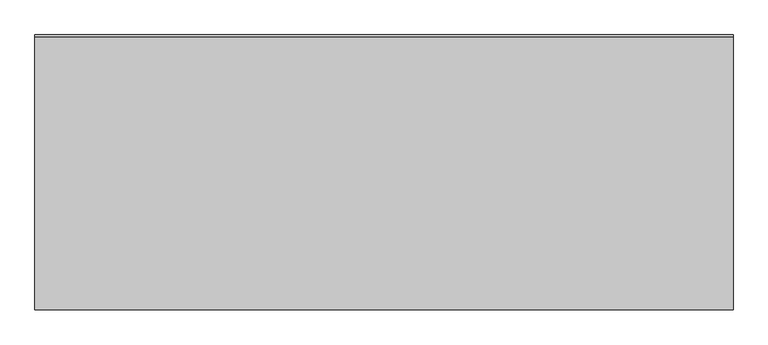
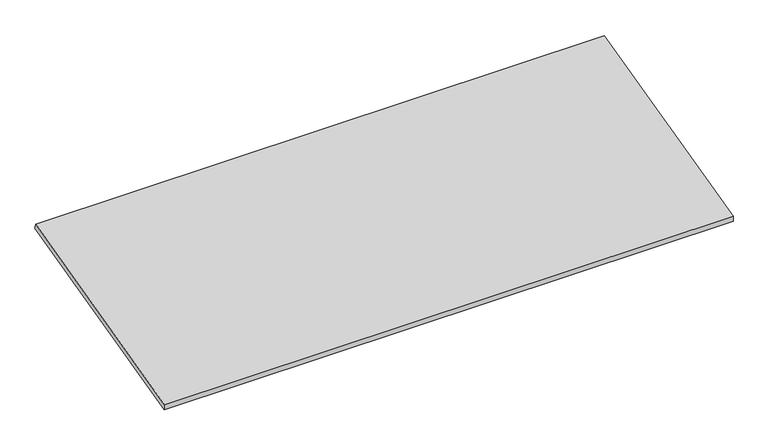
"""IFC4 building model written with IfcOpenShell, lengths in millimetres: proxy geometry, Plywood010 981 : Plywood010 981."""

from ifc_helpers import new_model, si_unit, frame, origin, place, context, project, spatial, polyline, outline, extrude, source, transform, mapped, element, save


def generic_models_1322f4c4(model_context):
    return source(origin(), model_context, "Body", "SweptSolid", [
        extrude(outline(polyline([(9641.0726949, 43605.6681404), (9645.7129487, 43587.1122956), (8857.883325, 43390.1000073), (8857.883325, 43409.7366198), (9641.0726949, 43605.6681404)])), frame((3694.2883192, 0.0, 0.0), z_axis=(1.0, 0.0, 0.0), x_axis=(0.0, 1.0, 0.0)), (0.0, 0.0, 1.0), 2000.0),
    ])


if __name__ == "__main__":
    model = new_model("IFC4")
    model_context = context("Model", 3, world=origin())
    ifc_project = project(units=[si_unit("LENGTHUNIT", "METRE", prefix="MILLI")], contexts=[model_context])
    site = spatial("IfcSite", under=ifc_project)
    building = spatial("IfcBuilding", under=site)
    placement = place(None, origin())
    generic_models_shape = generic_models_1322f4c4(model_context)
    element("IfcBuildingElementProxy", 1, Name="Plywood010 981 : Plywood010 981", ObjectType="Plywood010 981 : Plywood010 981", at=placement, inside=building, context=model_context, shape_type="MappedRepresentation", body=[
        mapped(generic_models_shape, transform((0.0, 0.0, 0.0), x_axis=(1.0, 0.0, 0.0), y_axis=(0.0, 1.0, 0.0), z_axis=(0.0, 0.0, 1.0))),
    ])
    save(model, "model.ifc")

# Revit data of these elements
# Type "Plywood010 981 : Plywood010 981"
#   NameOverride = "Plywood010"
# Element 1 (IfcBuildingElementProxy, "Plywood010 981 : Plywood010 981")
#   Materials on its faces: "CDX PLYWOOD - SEE STRUCTURAL DWGS"
# Materials
#   "CDX PLYWOOD - SEE STRUCTURAL DWGS": class "Unassigned", colour RGB 177 130 114, transparency 0, Cost = 0
